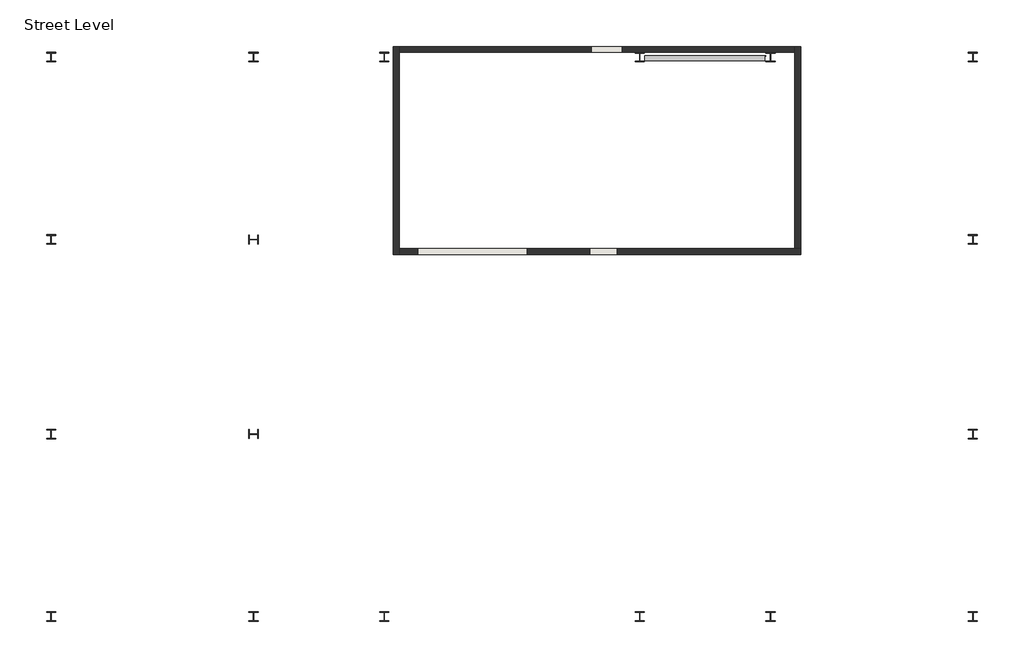
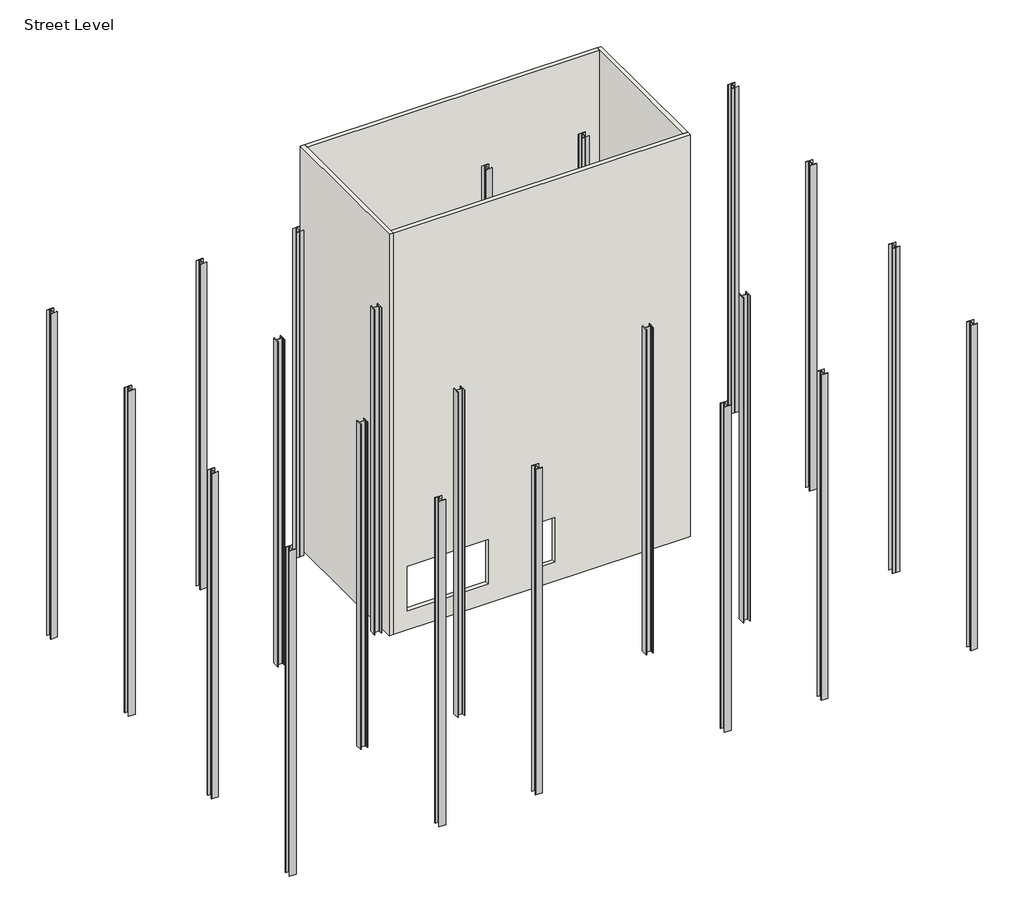
# One storey: 24 columns, 4 walls, 1 member.
"""IFC4 building model written with IfcOpenShell, lengths in millimetres."""

import ifcopenshell
import ifcopenshell.guid

model = None  # the IFC model being written
_history = None  # IfcOwnerHistory: only IFC2X3 demands one
_inside = {}  # id of a spatial element -> (the spatial element, [elements in it])
_under = {}  # id of a project, library or spatial element -> (it, [spatial elements below it])
_declared = {}  # id of a project -> (the project, [libraries it declares])
_typed = {}  # id of a type object -> (the type object, [elements of that type])
_made_of = {}  # id of a material, layer set ... -> (it, [elements and type objects made of it])


def new_model(schema):
    """Start an empty IFC model of exactly this schema.

    Asked for "IFC4X3", IfcOpenShell would pick the latest addendum, in which some entities
    have other attributes; the version numbers below select the first issue.
    IFC2X3 requires an IfcOwnerHistory on every rooted entity: one is made here for all.
    """
    global model, _history
    if schema == "IFC4X3":
        model = ifcopenshell.file(schema_version=(4, 3, 0, 0))
    else:
        model = ifcopenshell.file(schema=schema)
    _inside.clear()
    _under.clear()
    _declared.clear()
    _typed.clear()
    _made_of.clear()
    _history = None
    if model.schema == "IFC2X3":
        org = make("IfcOrganization", Name="unknown")
        user = make(
            "IfcPersonAndOrganization",
            ThePerson=make("IfcPerson", FamilyName="unknown"),
            TheOrganization=org,
        )
        app = make(
            "IfcApplication",
            ApplicationDeveloper=org,
            Version="unknown",
            ApplicationFullName="unknown",
            ApplicationIdentifier="unknown",
        )
        _history = make(
            "IfcOwnerHistory",
            OwningUser=user,
            OwningApplication=app,
            ChangeAction="ADDED",
            CreationDate=0,
        )
    return model


def make(cls, **values):
    """One entity of the class cls with the attributes given. An attribute that is None is left unset."""
    return model.create_entity(
        cls, **{name: value for name, value in values.items() if value is not None}
    )


def rooted(cls, **values):
    """An entity with a GlobalId (a new one), such as an element, a storey or a relation."""
    return make(cls, GlobalId=ifcopenshell.guid.new(), OwnerHistory=_history, **values)


def si_unit(unit_type, name, prefix=None):
    """IfcSIUnit, for example si_unit("LENGTHUNIT", "METRE", prefix="MILLI")."""
    return make("IfcSIUnit", UnitType=unit_type, Prefix=prefix, Name=name)


def assignment(units):
    """IfcUnitAssignment: the units of a project."""
    return None if units is None else make("IfcUnitAssignment", Units=units)


def point(xyz):
    """IfcCartesianPoint."""
    return None if xyz is None else make("IfcCartesianPoint", Coordinates=xyz)


def direction(xyz):
    """IfcDirection."""
    return None if xyz is None else make("IfcDirection", DirectionRatios=xyz)


def frame(location, z_axis=None, x_axis=None):
    """IfcAxis2Placement3D, a coordinate frame: its origin and axes. An axis left out is left unset."""
    return make(
        "IfcAxis2Placement3D",
        Location=point(location),
        Axis=direction(z_axis),
        RefDirection=direction(x_axis),
    )


def frame_2d(location, x_axis=None):
    """IfcAxis2Placement2D, a coordinate frame in the plane: its origin and x axis."""
    return make(
        "IfcAxis2Placement2D", Location=point(location), RefDirection=direction(x_axis)
    )


def origin():
    """The frame at (0, 0, 0) with its axes left unset."""
    return frame((0.0, 0.0, 0.0))


def place(relative_to, where):
    """IfcLocalPlacement: puts the frame where relative to a parent placement (None: the world)."""
    return make(
        "IfcLocalPlacement", PlacementRelTo=relative_to, RelativePlacement=where
    )


def context(
    kind, dimensions, precision=None, world=None, true_north=None, identifier=None
):
    """IfcGeometricRepresentationContext, for example the 3D "Model" context."""
    return make(
        "IfcGeometricRepresentationContext",
        ContextIdentifier=identifier,
        ContextType=kind,
        CoordinateSpaceDimension=dimensions,
        Precision=precision,
        WorldCoordinateSystem=world,
        TrueNorth=true_north,
    )


def project(units=None, contexts=None):
    """IfcProject with its units and contexts."""
    return rooted(
        "IfcProject",
        Name="project",
        RepresentationContexts=contexts,
        UnitsInContext=assignment(units),
    )


def spatial(cls, under=None, at=None, **own):
    """A site, building, storey or space (cls), placed at a placement, below another one or the project."""
    s = rooted(cls, ObjectPlacement=at, **own)
    if under is not None:
        _under.setdefault(under.id(), (under, []))[1].append(s)
    return s


def polyline(points):
    """IfcPolyline through the points."""
    return make("IfcPolyline", Points=[point(p) for p in points])


def circle_curve(where, radius):
    """IfcCircle in the frame where."""
    return make("IfcCircle", Position=where, Radius=radius)


def trimmed(basis, trim1, trim2, sense, master):
    """IfcTrimmedCurve: the piece of a basis curve between two trims."""
    return make(
        "IfcTrimmedCurve",
        BasisCurve=basis,
        Trim1=trim1,
        Trim2=trim2,
        SenseAgreement=sense,
        MasterRepresentation=master,
    )


def segment(curve, same_sense, transition):
    """IfcCompositeCurveSegment."""
    return make(
        "IfcCompositeCurveSegment",
        Transition=transition,
        SameSense=same_sense,
        ParentCurve=curve,
    )


def composite_curve(segments, self_intersect=None):
    """IfcCompositeCurve: segments joined end to end."""
    return make("IfcCompositeCurve", Segments=segments, SelfIntersect=self_intersect)


def outline(outer, holes=None, kind="AREA"):
    """IfcArbitraryClosedProfileDef: a profile drawn as a closed curve; with holes, ...WithVoids."""
    if holes is None:
        return make("IfcArbitraryClosedProfileDef", ProfileType=kind, OuterCurve=outer)
    return make(
        "IfcArbitraryProfileDefWithVoids",
        ProfileType=kind,
        OuterCurve=outer,
        InnerCurves=holes,
    )


def extrude(swept, where, along, depth):
    """IfcExtrudedAreaSolid: the profile swept, set in the frame where, extruded along a direction by depth."""
    return make(
        "IfcExtrudedAreaSolid",
        SweptArea=swept,
        Position=where,
        ExtrudedDirection=direction(along),
        Depth=depth,
    )


def faces_of(points, faces, orient=None, outer=None):
    """IfcFace entities. A face is a list of loops; a loop is a list of indices into points, from 0.

    orient and outer hold one flag for each loop. By default every Orientation is true, the
    first loop of a face is its IfcFaceOuterBound and the others are IfcFaceBound.
    """
    made = []
    for i, loops in enumerate(faces):
        bounds = []
        for j, loop in enumerate(loops):
            is_outer = j == 0 if outer is None else outer[i][j]
            bounds.append(
                make(
                    "IfcFaceOuterBound" if is_outer else "IfcFaceBound",
                    Bound=make("IfcPolyLoop", Polygon=[points[k] for k in loop]),
                    Orientation=True if orient is None else orient[i][j],
                )
            )
        made.append(make("IfcFace", Bounds=bounds))
    return made


def faceted_brep(points, faces, orient=None, outer=None, voids=None):
    """IfcFacetedBrep: a solid bounded by flat faces; with voids (closed shells), ...WithVoids."""
    shared = [point(p) for p in points]
    hull = make("IfcClosedShell", CfsFaces=faces_of(shared, faces, orient, outer))
    if voids is None:
        return make("IfcFacetedBrep", Outer=hull)
    return make(
        "IfcFacetedBrepWithVoids",
        Outer=hull,
        Voids=[
            make(cls, CfsFaces=faces_of(shared, fs, o, b)) for cls, fs, o, b in voids
        ],
    )


def shape(context_of_items, identifier, shape_type, items):
    """IfcShapeRepresentation: the items that make up one representation, for example the "Body"."""
    return make(
        "IfcShapeRepresentation",
        ContextOfItems=context_of_items,
        RepresentationIdentifier=identifier,
        RepresentationType=shape_type,
        Items=items,
    )


def source(mapping_origin, context_of_items, identifier, shape_type, items):
    """IfcRepresentationMap: a shape defined once, which mapped items show again and again."""
    return make(
        "IfcRepresentationMap",
        MappingOrigin=mapping_origin,
        MappedRepresentation=shape(context_of_items, identifier, shape_type, items),
    )


def transform(
    local_origin,
    x_axis=None,
    y_axis=None,
    z_axis=None,
    scale=None,
    scale2=None,
    scale3=None,
    uniform=True,
):
    """IfcCartesianTransformationOperator3D, or its non-uniform kind. x_axis, y_axis, z_axis: its Axis1, 2, 3."""
    if uniform:
        return make(
            "IfcCartesianTransformationOperator3D",
            Axis1=direction(x_axis),
            Axis2=direction(y_axis),
            LocalOrigin=point(local_origin),
            Scale=scale,
            Axis3=direction(z_axis),
        )
    return make(
        "IfcCartesianTransformationOperator3DnonUniform",
        Axis1=direction(x_axis),
        Axis2=direction(y_axis),
        LocalOrigin=point(local_origin),
        Scale=scale,
        Axis3=direction(z_axis),
        Scale2=scale2,
        Scale3=scale3,
    )


def mapped(mapping_source, mapping_target):
    """IfcMappedItem: shows the shape of a source again, moved by a transform."""
    return make(
        "IfcMappedItem", MappingSource=mapping_source, MappingTarget=mapping_target
    )


def made_of(thing, what):
    """Note that an element or type object is made of a material, layer set ...; save() writes the relation."""
    if what is not None:
        _made_of.setdefault(what.id(), (what, []))[1].append(thing)
    return thing


def element(
    cls,
    number,
    at=None,
    inside=None,
    cuts=None,
    type_object=None,
    material=None,
    context=None,
    identifier="Body",
    shape_type=None,
    held_by="IfcProductDefinitionShape",
    body=None,
    shapes=None,
    **own,
):
    """One element of the class cls, such as IfcWall. Its Tag is "e" and its number.

    at: its placement. inside: the storey or other place that contains it. cuts: it is an
    opening in that element (IfcRelVoidsElement). A single representation is given by context,
    identifier, shape_type and body (its items); several are given by shapes. held_by: the class
    of the entity that holds the representations. save() writes the other relations.
    """
    e = rooted(cls, Tag="e%d" % number, ObjectPlacement=at, **own)
    if body is not None:
        shapes = [shape(context, identifier, shape_type, body)]
    if shapes is not None:
        e.Representation = make(held_by, Representations=shapes)
    if inside is not None:
        _inside.setdefault(inside.id(), (inside, []))[1].append(e)
    if cuts is not None:
        rooted(
            "IfcRelVoidsElement", RelatingBuildingElement=cuts, RelatedOpeningElement=e
        )
    if type_object is not None:
        _typed.setdefault(type_object.id(), (type_object, []))[1].append(e)
    return made_of(e, material)


def aggregate(whole, parts):
    """IfcRelAggregates: a whole, such as a stair, and the parts it consists of."""
    return rooted("IfcRelAggregates", RelatingObject=whole, RelatedObjects=parts)


def save(model, path):
    """Write the relations noted so far, then the file.

    IfcRelAggregates (storeys below a building ...), IfcRelContainedInSpatialStructure (elements
    in a storey), IfcRelDefinesByType, IfcRelAssociatesMaterial and IfcRelDeclares: one each for
    every whole, place, type object, material and project.
    """
    for whole, parts in _under.values():
        aggregate(whole, parts)
    for where, things in _inside.values():
        rooted(
            "IfcRelContainedInSpatialStructure",
            RelatedElements=things,
            RelatingStructure=where,
        )
    for kind, things in _typed.values():
        rooted("IfcRelDefinesByType", RelatedObjects=things, RelatingType=kind)
    for what, things in _made_of.values():
        rooted("IfcRelAssociatesMaterial", RelatedObjects=things, RelatingMaterial=what)
    for by, libraries in _declared.values():
        rooted("IfcRelDeclares", RelatingContext=by, RelatedDefinitions=libraries)
    model.write(path)


def w_wide_flange_column_w12x87_da20b1fb(model_context):
    return source(origin(), model_context, "Body", "SweptSolid", [
        extrude(outline(composite_curve([segment(polyline([(153.9875, 159.146875), (153.9875, 138.6085937), (28.8726562, 138.6085937)]), True, "CONTINUOUS"), segment(trimmed(circle_curve(frame_2d((28.8726562, 116.284375)), 22.3242188), [point((28.8726562, 138.6085937))], [point((6.5484375, 116.284375))], True, "CARTESIAN"), True, "CONTINUOUS"), segment(polyline([(6.5484375, 116.284375), (6.5484375, -116.284375)]), True, "CONTINUOUS"), segment(trimmed(circle_curve(frame_2d((28.8726562, -116.284375)), 22.3242188), [point((6.5484375, -116.284375))], [point((28.8726562, -138.6085937))], True, "CARTESIAN"), True, "CONTINUOUS"), segment(polyline([(28.8726562, -138.6085937), (153.9875, -138.6085937), (153.9875, -159.146875), (-153.9875, -159.146875), (-153.9875, -138.6085937), (-28.8726563, -138.6085937)]), True, "CONTINUOUS"), segment(trimmed(circle_curve(frame_2d((-28.8726563, -116.284375)), 22.3242188), [point((-28.8726563, -138.6085937))], [point((-6.5484375, -116.284375))], True, "CARTESIAN"), True, "CONTINUOUS"), segment(polyline([(-6.5484375, -116.284375), (-6.5484375, 116.284375)]), True, "CONTINUOUS"), segment(trimmed(circle_curve(frame_2d((-28.8726563, 116.284375)), 22.3242188), [point((-6.5484375, 116.284375))], [point((-28.8726563, 138.6085937))], True, "CARTESIAN"), True, "CONTINUOUS"), segment(polyline([(-28.8726563, 138.6085937), (-153.9875, 138.6085937), (-153.9875, 159.146875), (153.9875, 159.146875)]), True, "CONTINUOUS")], self_intersect=False)), frame((0.0, 0.0, -914.4), z_axis=(0.0, 0.0, 1.0), x_axis=(1.0, 0.0, 0.0)), (0.0, 0.0, 1.0), 15544.8),
    ])


def l_angle2_l6x6x3_8_670392f0(model_context):
    return source(origin(), model_context, "Body", "SweptSolid", [
        extrude(outline(composite_curve([segment(polyline([(41.148, 41.148), (41.148, -111.252)]), True, "CONTINUOUS"), segment(trimmed(circle_curve(frame_2d((41.148, -101.727)), 9.525), [point((41.148, -111.252))], [point((31.623, -101.727))], False, "CARTESIAN"), True, "CONTINUOUS"), segment(polyline([(31.623, -101.727), (31.623, 22.098)]), True, "CONTINUOUS"), segment(trimmed(circle_curve(frame_2d((22.098, 22.098)), 9.525), [point((31.623, 22.098))], [point((22.098, 31.623))], True, "CARTESIAN"), True, "CONTINUOUS"), segment(polyline([(22.098, 31.623), (-101.727, 31.623)]), True, "CONTINUOUS"), segment(trimmed(circle_curve(frame_2d((-101.727, 41.148)), 9.525), [point((-101.727, 31.623))], [point((-111.252, 41.148))], False, "CARTESIAN"), True, "CONTINUOUS"), segment(polyline([(-111.252, 41.148), (41.148, 41.148)]), True, "CONTINUOUS")], self_intersect=False)), frame((-2053.0970548, 0.0, 0.0), z_axis=(1.0, 0.0, 0.0), x_axis=(0.0, 1.0, 0.0)), (0.0, 0.0, 1.0), 4091.5211794),
    ])


model = new_model("IFC4")

# Units and contexts
model_context = context("Model", 3, world=origin())
ifc_project = project(units=[si_unit("LENGTHUNIT", "METRE", prefix="MILLI")], contexts=[model_context])

# Site, building, storey
site = spatial("IfcSite", under=ifc_project)
building = spatial("IfcBuilding", under=site)
storey = spatial("IfcBuildingStorey", under=building, Name="Street Level", Elevation=-914.4)

# Columns
placement = place(None, origin())
w_wide_flange_column_w12x87_shape = w_wide_flange_column_w12x87_da20b1fb(model_context)
element("IfcColumn", 1, ObjectType="W-Wide Flange-Column : W12X87", at=placement, inside=storey, context=model_context, shape_type="MappedRepresentation", body=[
    mapped(w_wide_flange_column_w12x87_shape, transform((-9801.8122732, -3408.4984696, 0.0), x_axis=(0.0, -1.0, 0.0), y_axis=(1.0, 0.0, 0.0), z_axis=(0.0, 0.0, 1.0))),
])
element("IfcColumn", 2, ObjectType="W-Wide Flange-Column : W12X87", at=placement, inside=storey, context=model_context, shape_type="MappedRepresentation", body=[
    mapped(w_wide_flange_column_w12x87_shape, transform((-5433.0122732, -3408.4984696, 0.0), x_axis=(0.0, -1.0, 0.0), y_axis=(1.0, 0.0, 0.0), z_axis=(0.0, 0.0, 1.0))),
])
element("IfcColumn", 3, ObjectType="W-Wide Flange-Column : W12X87", at=placement, inside=storey, context=model_context, shape_type="MappedRepresentation", body=[
    mapped(w_wide_flange_column_w12x87_shape, transform((3101.3877268, -3408.4984696, 0.0), x_axis=(0.0, -1.0, 0.0), y_axis=(1.0, 0.0, 0.0), z_axis=(0.0, 0.0, 1.0))),
])
element("IfcColumn", 4, ObjectType="W-Wide Flange-Column : W12X87", at=placement, inside=storey, context=model_context, shape_type="MappedRepresentation", body=[
    mapped(w_wide_flange_column_w12x87_shape, transform((7470.1877268, -3408.4984696, 0.0), x_axis=(0.0, -1.0, 0.0), y_axis=(1.0, 0.0, 0.0), z_axis=(0.0, 0.0, 1.0))),
])
element("IfcColumn", 5, ObjectType="W-Wide Flange-Column : W12X87", at=placement, inside=storey, context=model_context, shape_type="MappedRepresentation", body=[
    mapped(w_wide_flange_column_w12x87_shape, transform((-9801.8122732, 3093.9015304, 0.0), x_axis=(0.0, -1.0, 0.0), y_axis=(1.0, 0.0, 0.0), z_axis=(0.0, 0.0, 1.0))),
])
element("IfcColumn", 6, ObjectType="W-Wide Flange-Column : W12X87", at=placement, inside=storey, context=model_context, shape_type="MappedRepresentation", body=[
    mapped(w_wide_flange_column_w12x87_shape, transform((-5433.0122732, 3093.9015304, 0.0), x_axis=(0.0, -1.0, 0.0), y_axis=(1.0, 0.0, 0.0), z_axis=(0.0, 0.0, 1.0))),
])
element("IfcColumn", 7, ObjectType="W-Wide Flange-Column : W12X87", at=placement, inside=storey, context=model_context, shape_type="MappedRepresentation", body=[
    mapped(w_wide_flange_column_w12x87_shape, transform((3101.3877268, 3093.9015304, 0.0), x_axis=(0.0, -1.0, 0.0), y_axis=(1.0, 0.0, 0.0), z_axis=(0.0, 0.0, 1.0))),
])
element("IfcColumn", 8, ObjectType="W-Wide Flange-Column : W12X87", at=placement, inside=storey, context=model_context, shape_type="MappedRepresentation", body=[
    mapped(w_wide_flange_column_w12x87_shape, transform((7470.1877268, 3093.9015304, 0.0), x_axis=(0.0, -1.0, 0.0), y_axis=(1.0, 0.0, 0.0), z_axis=(0.0, 0.0, 1.0))),
])
element("IfcColumn", 9, ObjectType="W-Wide Flange-Column : W12X87", at=placement, inside=storey, context=model_context, shape_type="MappedRepresentation", body=[
    mapped(w_wide_flange_column_w12x87_shape, transform((-16558.2122732, 9189.9015304, 0.0), x_axis=(1.0, 0.0, 0.0), y_axis=(0.0, 1.0, 0.0), z_axis=(0.0, 0.0, 1.0))),
])
element("IfcColumn", 10, ObjectType="W-Wide Flange-Column : W12X87", at=placement, inside=storey, context=model_context, shape_type="MappedRepresentation", body=[
    mapped(w_wide_flange_column_w12x87_shape, transform((-16558.2122732, 3093.9015304, 0.0), x_axis=(1.0, 0.0, 0.0), y_axis=(0.0, 1.0, 0.0), z_axis=(0.0, 0.0, 1.0))),
])
element("IfcColumn", 11, ObjectType="W-Wide Flange-Column : W12X87", at=placement, inside=storey, context=model_context, shape_type="MappedRepresentation", body=[
    mapped(w_wide_flange_column_w12x87_shape, transform((-9801.8122732, 9189.9015304, 0.0), x_axis=(1.0, 0.0, 0.0), y_axis=(0.0, 1.0, 0.0), z_axis=(0.0, 0.0, 1.0))),
])
element("IfcColumn", 12, ObjectType="W-Wide Flange-Column : W12X87", at=placement, inside=storey, context=model_context, shape_type="MappedRepresentation", body=[
    mapped(w_wide_flange_column_w12x87_shape, transform((-5433.0122732, 9189.9015304, 0.0), x_axis=(1.0, 0.0, 0.0), y_axis=(0.0, 1.0, 0.0), z_axis=(0.0, 0.0, 1.0))),
])
element("IfcColumn", 13, ObjectType="W-Wide Flange-Column : W12X87", at=placement, inside=storey, context=model_context, shape_type="MappedRepresentation", body=[
    mapped(w_wide_flange_column_w12x87_shape, transform((3101.3877268, 9189.9015304, 0.0), x_axis=(1.0, 0.0, 0.0), y_axis=(0.0, 1.0, 0.0), z_axis=(0.0, 0.0, 1.0))),
])
element("IfcColumn", 14, ObjectType="W-Wide Flange-Column : W12X87", at=placement, inside=storey, context=model_context, shape_type="MappedRepresentation", body=[
    mapped(w_wide_flange_column_w12x87_shape, transform((7470.1877268, 9189.9015304, 0.0), x_axis=(1.0, 0.0, 0.0), y_axis=(0.0, 1.0, 0.0), z_axis=(0.0, 0.0, 1.0))),
])
element("IfcColumn", 15, ObjectType="W-Wide Flange-Column : W12X87", at=placement, inside=storey, context=model_context, shape_type="MappedRepresentation", body=[
    mapped(w_wide_flange_column_w12x87_shape, transform((14226.5877268, 9189.9015304, 0.0), x_axis=(1.0, 0.0, 0.0), y_axis=(0.0, 1.0, 0.0), z_axis=(0.0, 0.0, 1.0))),
])
element("IfcColumn", 16, ObjectType="W-Wide Flange-Column : W12X87", at=placement, inside=storey, context=model_context, shape_type="MappedRepresentation", body=[
    mapped(w_wide_flange_column_w12x87_shape, transform((14226.5877268, 3093.9015304, 0.0), x_axis=(1.0, 0.0, 0.0), y_axis=(0.0, 1.0, 0.0), z_axis=(0.0, 0.0, 1.0))),
])
element("IfcColumn", 17, ObjectType="W-Wide Flange-Column : W12X87", at=placement, inside=storey, context=model_context, shape_type="MappedRepresentation", body=[
    mapped(w_wide_flange_column_w12x87_shape, transform((14226.5877268, -3408.4984696, 0.0), x_axis=(1.0, 0.0, 0.0), y_axis=(0.0, 1.0, 0.0), z_axis=(0.0, 0.0, 1.0))),
])
element("IfcColumn", 18, ObjectType="W-Wide Flange-Column : W12X87", at=placement, inside=storey, context=model_context, shape_type="MappedRepresentation", body=[
    mapped(w_wide_flange_column_w12x87_shape, transform((14226.5877268, -9504.4984696, 0.0), x_axis=(1.0, 0.0, 0.0), y_axis=(0.0, 1.0, 0.0), z_axis=(0.0, 0.0, 1.0))),
])
element("IfcColumn", 19, ObjectType="W-Wide Flange-Column : W12X87", at=placement, inside=storey, context=model_context, shape_type="MappedRepresentation", body=[
    mapped(w_wide_flange_column_w12x87_shape, transform((7470.1877268, -9504.4984696, 0.0), x_axis=(1.0, 0.0, 0.0), y_axis=(0.0, 1.0, 0.0), z_axis=(0.0, 0.0, 1.0))),
])
element("IfcColumn", 20, ObjectType="W-Wide Flange-Column : W12X87", at=placement, inside=storey, context=model_context, shape_type="MappedRepresentation", body=[
    mapped(w_wide_flange_column_w12x87_shape, transform((3101.3877268, -9504.4984696, 0.0), x_axis=(1.0, 0.0, 0.0), y_axis=(0.0, 1.0, 0.0), z_axis=(0.0, 0.0, 1.0))),
])
element("IfcColumn", 21, ObjectType="W-Wide Flange-Column : W12X87", at=placement, inside=storey, context=model_context, shape_type="MappedRepresentation", body=[
    mapped(w_wide_flange_column_w12x87_shape, transform((-5433.0122732, -9504.4984696, 0.0), x_axis=(1.0, 0.0, 0.0), y_axis=(0.0, 1.0, 0.0), z_axis=(0.0, 0.0, 1.0))),
])
element("IfcColumn", 22, ObjectType="W-Wide Flange-Column : W12X87", at=placement, inside=storey, context=model_context, shape_type="MappedRepresentation", body=[
    mapped(w_wide_flange_column_w12x87_shape, transform((-9801.8122732, -9504.4984696, 0.0), x_axis=(1.0, 0.0, 0.0), y_axis=(0.0, 1.0, 0.0), z_axis=(0.0, 0.0, 1.0))),
])
element("IfcColumn", 23, ObjectType="W-Wide Flange-Column : W12X87", at=placement, inside=storey, context=model_context, shape_type="MappedRepresentation", body=[
    mapped(w_wide_flange_column_w12x87_shape, transform((-16558.2122732, -9504.4984696, 0.0), x_axis=(1.0, 0.0, 0.0), y_axis=(0.0, 1.0, 0.0), z_axis=(0.0, 0.0, 1.0))),
])
element("IfcColumn", 24, ObjectType="W-Wide Flange-Column : W12X87", at=placement, inside=storey, context=model_context, shape_type="MappedRepresentation", body=[
    mapped(w_wide_flange_column_w12x87_shape, transform((-16558.2122732, -3408.4984696, 0.0), x_axis=(1.0, 0.0, 0.0), y_axis=(0.0, 1.0, 0.0), z_axis=(0.0, 0.0, 1.0))),
])

# Member
l_angle2_l6x6x3_8_shape = l_angle2_l6x6x3_8_670392f0(model_context)
element("IfcMember", 25, ObjectType="L-Angle2 : L6X6X3/8", at=placement, inside=storey, context=model_context, shape_type="MappedRepresentation", body=[
    mapped(l_angle2_l6x6x3_8_shape, transform((5285.7877268, 9189.9015304, -457.2), x_axis=(0.9787906252528689, 0.0, 0.20486315412269337), y_axis=(0.0, 1.0000000000000002, 0.0), z_axis=(-0.20486315412269337, 0.0, 0.9787906252528689))),
])

# Walls
element("IfcWall", 26, ObjectType="Generic - 8\" Masonry", at=placement, inside=storey, context=model_context, shape_type="Brep", body=[
    faceted_brep([(-5128.2122732, 9545.5015304, -914.4), (-5128.2122732, 2595.4265304, -914.4), (-5128.2122732, 2595.4265304, 18288.0), (-5128.2122732, 9545.5015304, 18288.0), (-4934.5372732, 9545.5015304, -914.4), (-4934.5372732, 9545.5015304, 18288.0), (-4934.5372732, 9351.8265304, 18288.0), (-4934.5372732, 2789.1015304, 18288.0), (-4934.5372732, 2595.4265304, 18288.0), (-4934.5372732, 2595.4265304, -914.4), (-4934.5372732, 2789.1015304, -914.4), (-4934.5372732, 9351.8265304, -914.4)], [[[0, 1, 2, 3]], [[4, 5, 6, 7, 8, 9, 10, 11]], [[1, 0, 4, 11, 10, 9]], [[3, 2, 8, 7, 6, 5]], [[0, 3, 5, 4]], [[2, 1, 9, 8]]]),
])
element("IfcWall", 27, ObjectType="Generic - 8\" Masonry", at=placement, inside=storey, context=model_context, shape_type="Brep", body=[
    faceted_brep([(8476.6627268, 2789.1015304, -914.4), (8282.9877268, 2789.1015304, -914.4), (-4934.5372732, 2789.1015304, -914.4), (-4934.5372732, 2789.1015304, 18288.0), (8282.9877268, 2789.1015304, 18288.0), (8476.6627268, 2789.1015304, 18288.0), (-653.0497732, 2789.1015304, 2133.6), (-4310.6497732, 2789.1015304, 2133.6), (-4310.6497732, 2789.1015304, 0.0), (-653.0497732, 2789.1015304, 0.0), (2344.1502268, 2789.1015304, 2133.6), (1429.7502268, 2789.1015304, 2133.6), (1429.7502268, 2789.1015304, 0.0), (2344.1502268, 2789.1015304, 0.0), (-4934.5372732, 2595.4265304, -914.4), (8476.6627268, 2595.4265304, -914.4), (8476.6627268, 2595.4265304, 18288.0), (-4934.5372732, 2595.4265304, 18288.0), (-4310.6497732, 2595.4265304, 2133.6), (-653.0497732, 2595.4265304, 2133.6), (-653.0497732, 2595.4265304, 0.0), (-4310.6497732, 2595.4265304, 0.0), (1429.7502268, 2595.4265304, 2133.6), (2344.1502268, 2595.4265304, 2133.6), (2344.1502268, 2595.4265304, 0.0), (1429.7502268, 2595.4265304, 0.0)], [[[0, 1, 2, 3, 4, 5], [6, 7, 8, 9], [10, 11, 12, 13]], [[14, 15, 16, 17], [18, 19, 20, 21], [22, 23, 24, 25]], [[2, 1, 0, 15, 14]], [[5, 4, 3, 17, 16]], [[0, 5, 16, 15]], [[3, 2, 14, 17]], [[6, 19, 18, 7]], [[8, 21, 20, 9]], [[19, 6, 9, 20]], [[7, 18, 21, 8]], [[10, 23, 22, 11]], [[12, 25, 24, 13]], [[23, 10, 13, 24]], [[11, 22, 25, 12]]]),
])
element("IfcWall", 28, ObjectType="Generic - 8\" Masonry", at=placement, inside=storey, context=model_context, shape_type="Brep", body=[
    faceted_brep([(8282.9877268, 9545.5015304, -914.4), (8282.9877268, 9351.8265304, -914.4), (8282.9877268, 2789.1015304, -914.4), (8282.9877268, 2789.1015304, 18288.0), (8282.9877268, 9351.8265304, 18288.0), (8282.9877268, 9545.5015304, 18288.0), (8476.6627268, 9545.5015304, -914.4), (8476.6627268, 9545.5015304, 18288.0), (8476.6627268, 2789.1015304, 18288.0), (8476.6627268, 2789.1015304, -914.4)], [[[0, 1, 2, 3, 4, 5]], [[6, 7, 8, 9]], [[2, 1, 0, 6, 9]], [[5, 4, 3, 8, 7]], [[0, 5, 7, 6]], [[3, 2, 9, 8]]]),
])
element("IfcWall", 29, ObjectType="Generic - 8\" Masonry", at=placement, inside=storey, context=model_context, shape_type="SweptSolid", body=[
    extrude(outline(polyline([(-914.4, -4934.5372732), (-914.4, 8282.9877268), (18288.0, 8282.9877268), (18288.0, -4934.5372732), (-914.4, -4934.5372732)]), holes=[polyline([(2235.2, 1475.7877268), (2235.2, 2510.8377268), (0.0, 2510.8377268), (0.0, 1475.7877268), (2235.2, 1475.7877268)])]), frame((0.0, 9351.8265304, 0.0), z_axis=(0.0, 1.0, 0.0), x_axis=(0.0, 0.0, 1.0)), (0.0, 0.0, 1.0), 193.675),
])

save(model, "model.ifc")

# Revit data of these elements
# Project information
#   Organization Name = "G3B Press"
#   Organization Description = "Paul F. Aubin Cosulting Services, Inc."
#   Building Name = "Revit Essentials for Architecture"
#   Author = "Paul F. Aubin"
#   Author Website = "https://www.paulaubin.com"
#   Copyright = "Copyright © 2020 Paul F Aubin, all rights reserved"
#   Project Issue Date = "8/1/2020"
#   Project Status = "Design Development"
#   Client Name = "Vertical Circulation"
#   Project Address = "123 State ST\nSuite 301\nChicago, IL 60606"
#   Project Name = "08 Commercial-Structure_Complete"
#   Project Number = "2020.04S"
# Grids (mm)
#   "1": line (-22547.601, -9504.498) -> (19277.595, -9504.498)
#   "2": line (-22547.601, -3408.498) -> (19277.595, -3408.498)
#   "3": line (-22547.601, 3093.902) -> (19277.595, 3093.902)
#   "4": line (-22547.601, 9189.902) -> (19277.595, 9189.902)
#   "A": line (-16558.212, 12259.726) -> (-16558.212, -14197.104)
#   "B": line (-9801.812, 12259.726) -> (-9801.812, -14197.104)
#   "C": line (-5433.012, 12259.726) -> (-5433.012, -14197.104)
#   "D": line (3101.388, 12259.726) -> (3101.388, -14197.104)
#   "E": line (7470.188, 12259.726) -> (7470.188, -14197.104)
#   "F": line (14226.588, 12259.726) -> (14226.588, -14197.104)
#   "C.3": line (-2689.812, -15151.11) -> (-2689.812, -5965.346)
#   "C.7": line (358.188, -15151.11) -> (358.188, -5965.346)
# Type "W-Wide Flange-Column : W12X87"
#   Assembly Code = "B10"
#   A = 0.18 SF
#   W = 87
#   bf = 1' - 0 1/8"
#   d = 1' - 0 17/32"
#   k = 0' - 1 11/16"
#   kr = 0' - 0 225/256"
#   tf = 0' - 0 207/256"
#   tw = 0' - 0 33/64"
#   Structural Material [instance default] = Metal - Steel - ASTM A992
# Type "L-Angle2 : L6X6X3/8"
#   Assembly Code = "B10"
#   k = 0' - 0 7/8"
#   W = 14.9
#   Length [instance default] = 5' - 0"
#   b = 0' - 6"
#   d = 0' - 6"
#   t = 0' - 0 3/8"
#   x = 0' - 1.62"
#   y = 0' - 1.62"
#   A = 0.0304167 SF
#   Structural Material [instance default] = Steel ASTM A36
# Type "Generic - 8\" Masonry"
#   Assembly Code = "B2010"
#   Layers, outside or top first: 0' - 7 5/8" "Masonry - Concrete Masonry Units" (function 1)
# Elements 1, 2, 3, 4, 5, 6, 7, 8, 9, 10, 11, 12, 13, 14, 15, 16, 17, 18, 19, 20, 21, 22, 23, 24 (IfcColumn, "W-Wide Flange-Column : W12X87")
#   Structural Material = Metal - Steel - ASTM A992
#   Phase Created = New Construction
#   Materials on its faces: "Metal - Steel - ASTM A992"
# Element 25 (IfcMember, "L-Angle2 : L6X6X3/8")
#   Structural Material = Steel ASTM A36
#   Phase Created = New Construction
#   Materials on its faces: "Steel ASTM A36"
# Elements 26, 27, 28, 29 (IfcWall, "Generic - 8\" Masonry")
#   Top Offset = 12' - 0"
#   Base Offset = 0' - 0"
#   Unconnected Height = 63' - 0"
#   wall height = 63' - 0"
#   Phase Created = New Construction
#   Base Constraint = Street Level
#   Top Constraint = Roof
#   Materials on its faces: "Masonry - Concrete Masonry Units"
# Materials
#   "Metal - Steel - ASTM A992": class "Unassigned", colour RGB 199 199 199, transparency 0, Description = "Steel ASTM A992"
#   "Steel ASTM A36": class "Metal", colour RGB 199 199 199, transparency 0, Description = "Structural steel, ASTM A36 Grade B, mill finish", Cost = 0
#   "Masonry - Concrete Masonry Units": class "Unassigned", colour RGB 227 227 227, transparency 0, Description = "CMU"
